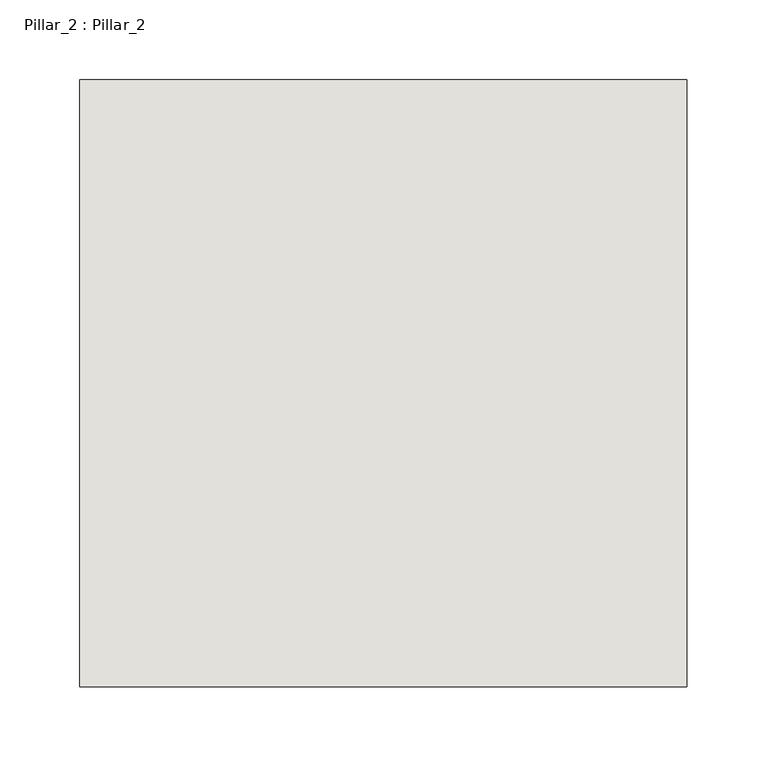
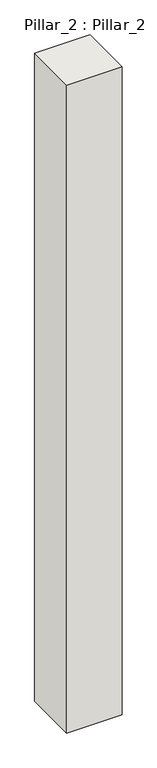
"""IFC4 building model written with IfcOpenShell, lengths in millimetres: wall geometry, Pillar_2 : Pillar_2."""

import ifcopenshell
import ifcopenshell.guid

model = None  # the IFC model being written
_history = None  # IfcOwnerHistory: only IFC2X3 demands one
_inside = {}  # id of a spatial element -> (the spatial element, [elements in it])
_under = {}  # id of a project, library or spatial element -> (it, [spatial elements below it])
_declared = {}  # id of a project -> (the project, [libraries it declares])
_typed = {}  # id of a type object -> (the type object, [elements of that type])
_made_of = {}  # id of a material, layer set ... -> (it, [elements and type objects made of it])


def new_model(schema):
    """Start an empty IFC model of exactly this schema.

    Asked for "IFC4X3", IfcOpenShell would pick the latest addendum, in which some entities
    have other attributes; the version numbers below select the first issue.
    IFC2X3 requires an IfcOwnerHistory on every rooted entity: one is made here for all.
    """
    global model, _history
    if schema == "IFC4X3":
        model = ifcopenshell.file(schema_version=(4, 3, 0, 0))
    else:
        model = ifcopenshell.file(schema=schema)
    _inside.clear()
    _under.clear()
    _declared.clear()
    _typed.clear()
    _made_of.clear()
    _history = None
    if model.schema == "IFC2X3":
        org = make("IfcOrganization", Name="unknown")
        user = make(
            "IfcPersonAndOrganization",
            ThePerson=make("IfcPerson", FamilyName="unknown"),
            TheOrganization=org,
        )
        app = make(
            "IfcApplication",
            ApplicationDeveloper=org,
            Version="unknown",
            ApplicationFullName="unknown",
            ApplicationIdentifier="unknown",
        )
        _history = make(
            "IfcOwnerHistory",
            OwningUser=user,
            OwningApplication=app,
            ChangeAction="ADDED",
            CreationDate=0,
        )
    return model


def make(cls, **values):
    """One entity of the class cls with the attributes given. An attribute that is None is left unset."""
    return model.create_entity(
        cls, **{name: value for name, value in values.items() if value is not None}
    )


def rooted(cls, **values):
    """An entity with a GlobalId (a new one), such as an element, a storey or a relation."""
    return make(cls, GlobalId=ifcopenshell.guid.new(), OwnerHistory=_history, **values)


def si_unit(unit_type, name, prefix=None):
    """IfcSIUnit, for example si_unit("LENGTHUNIT", "METRE", prefix="MILLI")."""
    return make("IfcSIUnit", UnitType=unit_type, Prefix=prefix, Name=name)


def assignment(units):
    """IfcUnitAssignment: the units of a project."""
    return None if units is None else make("IfcUnitAssignment", Units=units)


def point(xyz):
    """IfcCartesianPoint."""
    return None if xyz is None else make("IfcCartesianPoint", Coordinates=xyz)


def direction(xyz):
    """IfcDirection."""
    return None if xyz is None else make("IfcDirection", DirectionRatios=xyz)


def frame(location, z_axis=None, x_axis=None):
    """IfcAxis2Placement3D, a coordinate frame: its origin and axes. An axis left out is left unset."""
    return make(
        "IfcAxis2Placement3D",
        Location=point(location),
        Axis=direction(z_axis),
        RefDirection=direction(x_axis),
    )


def origin():
    """The frame at (0, 0, 0) with its axes left unset."""
    return frame((0.0, 0.0, 0.0))


def origin_with_axes():
    """The frame at (0, 0, 0) with the z axis (0, 0, 1) and the x axis (1, 0, 0) written out."""
    return frame((0.0, 0.0, 0.0), z_axis=(0.0, 0.0, 1.0), x_axis=(1.0, 0.0, 0.0))


def place(relative_to, where):
    """IfcLocalPlacement: puts the frame where relative to a parent placement (None: the world)."""
    return make(
        "IfcLocalPlacement", PlacementRelTo=relative_to, RelativePlacement=where
    )


def context(
    kind, dimensions, precision=None, world=None, true_north=None, identifier=None
):
    """IfcGeometricRepresentationContext, for example the 3D "Model" context."""
    return make(
        "IfcGeometricRepresentationContext",
        ContextIdentifier=identifier,
        ContextType=kind,
        CoordinateSpaceDimension=dimensions,
        Precision=precision,
        WorldCoordinateSystem=world,
        TrueNorth=true_north,
    )


def project(units=None, contexts=None):
    """IfcProject with its units and contexts."""
    return rooted(
        "IfcProject",
        Name="project",
        RepresentationContexts=contexts,
        UnitsInContext=assignment(units),
    )


def spatial(cls, under=None, at=None, **own):
    """A site, building, storey or space (cls), placed at a placement, below another one or the project."""
    s = rooted(cls, ObjectPlacement=at, **own)
    if under is not None:
        _under.setdefault(under.id(), (under, []))[1].append(s)
    return s


def polyline(points):
    """IfcPolyline through the points."""
    return make("IfcPolyline", Points=[point(p) for p in points])


def outline(outer, holes=None, kind="AREA"):
    """IfcArbitraryClosedProfileDef: a profile drawn as a closed curve; with holes, ...WithVoids."""
    if holes is None:
        return make("IfcArbitraryClosedProfileDef", ProfileType=kind, OuterCurve=outer)
    return make(
        "IfcArbitraryProfileDefWithVoids",
        ProfileType=kind,
        OuterCurve=outer,
        InnerCurves=holes,
    )


def extrude(swept, where, along, depth):
    """IfcExtrudedAreaSolid: the profile swept, set in the frame where, extruded along a direction by depth."""
    return make(
        "IfcExtrudedAreaSolid",
        SweptArea=swept,
        Position=where,
        ExtrudedDirection=direction(along),
        Depth=depth,
    )


def shape(context_of_items, identifier, shape_type, items):
    """IfcShapeRepresentation: the items that make up one representation, for example the "Body"."""
    return make(
        "IfcShapeRepresentation",
        ContextOfItems=context_of_items,
        RepresentationIdentifier=identifier,
        RepresentationType=shape_type,
        Items=items,
    )


def source(mapping_origin, context_of_items, identifier, shape_type, items):
    """IfcRepresentationMap: a shape defined once, which mapped items show again and again."""
    return make(
        "IfcRepresentationMap",
        MappingOrigin=mapping_origin,
        MappedRepresentation=shape(context_of_items, identifier, shape_type, items),
    )


def transform(
    local_origin,
    x_axis=None,
    y_axis=None,
    z_axis=None,
    scale=None,
    scale2=None,
    scale3=None,
    uniform=True,
):
    """IfcCartesianTransformationOperator3D, or its non-uniform kind. x_axis, y_axis, z_axis: its Axis1, 2, 3."""
    if uniform:
        return make(
            "IfcCartesianTransformationOperator3D",
            Axis1=direction(x_axis),
            Axis2=direction(y_axis),
            LocalOrigin=point(local_origin),
            Scale=scale,
            Axis3=direction(z_axis),
        )
    return make(
        "IfcCartesianTransformationOperator3DnonUniform",
        Axis1=direction(x_axis),
        Axis2=direction(y_axis),
        LocalOrigin=point(local_origin),
        Scale=scale,
        Axis3=direction(z_axis),
        Scale2=scale2,
        Scale3=scale3,
    )


def mapped(mapping_source, mapping_target):
    """IfcMappedItem: shows the shape of a source again, moved by a transform."""
    return make(
        "IfcMappedItem", MappingSource=mapping_source, MappingTarget=mapping_target
    )


def made_of(thing, what):
    """Note that an element or type object is made of a material, layer set ...; save() writes the relation."""
    if what is not None:
        _made_of.setdefault(what.id(), (what, []))[1].append(thing)
    return thing


def element(
    cls,
    number,
    at=None,
    inside=None,
    cuts=None,
    type_object=None,
    material=None,
    context=None,
    identifier="Body",
    shape_type=None,
    held_by="IfcProductDefinitionShape",
    body=None,
    shapes=None,
    **own,
):
    """One element of the class cls, such as IfcWall. Its Tag is "e" and its number.

    at: its placement. inside: the storey or other place that contains it. cuts: it is an
    opening in that element (IfcRelVoidsElement). A single representation is given by context,
    identifier, shape_type and body (its items); several are given by shapes. held_by: the class
    of the entity that holds the representations. save() writes the other relations.
    """
    e = rooted(cls, Tag="e%d" % number, ObjectPlacement=at, **own)
    if body is not None:
        shapes = [shape(context, identifier, shape_type, body)]
    if shapes is not None:
        e.Representation = make(held_by, Representations=shapes)
    if inside is not None:
        _inside.setdefault(inside.id(), (inside, []))[1].append(e)
    if cuts is not None:
        rooted(
            "IfcRelVoidsElement", RelatingBuildingElement=cuts, RelatedOpeningElement=e
        )
    if type_object is not None:
        _typed.setdefault(type_object.id(), (type_object, []))[1].append(e)
    return made_of(e, material)


def aggregate(whole, parts):
    """IfcRelAggregates: a whole, such as a stair, and the parts it consists of."""
    return rooted("IfcRelAggregates", RelatingObject=whole, RelatedObjects=parts)


def save(model, path):
    """Write the relations noted so far, then the file.

    IfcRelAggregates (storeys below a building ...), IfcRelContainedInSpatialStructure (elements
    in a storey), IfcRelDefinesByType, IfcRelAssociatesMaterial and IfcRelDeclares: one each for
    every whole, place, type object, material and project.
    """
    for whole, parts in _under.values():
        aggregate(whole, parts)
    for where, things in _inside.values():
        rooted(
            "IfcRelContainedInSpatialStructure",
            RelatedElements=things,
            RelatingStructure=where,
        )
    for kind, things in _typed.values():
        rooted("IfcRelDefinesByType", RelatedObjects=things, RelatingType=kind)
    for what, things in _made_of.values():
        rooted("IfcRelAssociatesMaterial", RelatedObjects=things, RelatingMaterial=what)
    for by, libraries in _declared.values():
        rooted("IfcRelDeclares", RelatingContext=by, RelatedDefinitions=libraries)
    model.write(path)


def pillar_2_pillar_2_c342d97b(model_context):
    return source(origin(), model_context, "Body", "SweptSolid", [
        extrude(outline(polyline([(240.0, 3770.0), (-140.0, 3770.0), (-140.0, 4150.0), (240.0, 4150.0), (240.0, 3770.0)])), origin_with_axes(), (0.0, 0.0, 1.0), 4700.0),
    ])


if __name__ == "__main__":
    model = new_model("IFC4")
    model_context = context("Model", 3, world=origin())
    ifc_project = project(units=[si_unit("LENGTHUNIT", "METRE", prefix="MILLI")], contexts=[model_context])
    site = spatial("IfcSite", under=ifc_project)
    building = spatial("IfcBuilding", under=site)
    placement = place(None, origin())
    pillar_2_pillar_2_shape = pillar_2_pillar_2_c342d97b(model_context)
    element("IfcWall", 1, ObjectType="Pillar_2 : Pillar_2", at=placement, inside=building, context=model_context, shape_type="MappedRepresentation", body=[
        mapped(pillar_2_pillar_2_shape, transform((0.0, 0.0, 0.0), x_axis=(1.0, 0.0, 0.0), y_axis=(0.0, 1.0, 0.0), z_axis=(0.0, 0.0, 1.0))),
    ])
    save(model, "model.ifc")

# Revit data of these elements
# Type "Pillar_2 : Pillar_2"
#   NameOverride = "Pillar_2"
# Element 1 (IfcWall, "Pillar_2 : Pillar_2")
#   Materials on its faces: "IfcSurfaceStyle #33"
# Materials
#   "IfcSurfaceStyle #33": class "Unassigned", colour RGB 214 214 214, transparency 0
